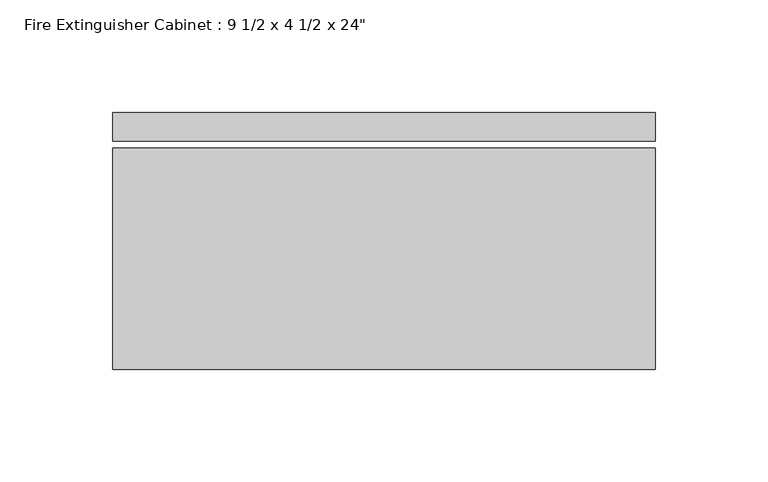
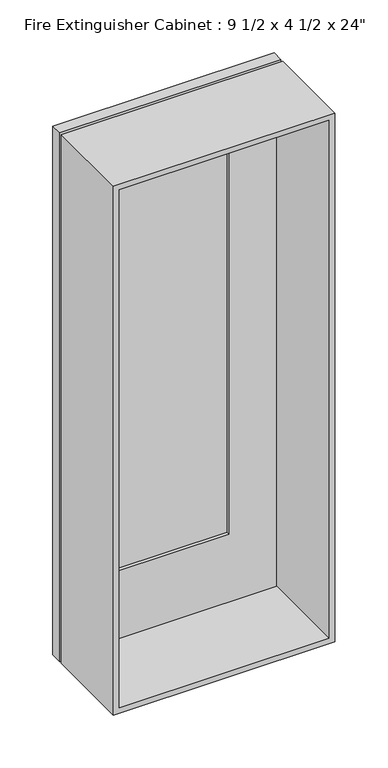
"""IFC4 building model written with IfcOpenShell, lengths in millimetres: proxy geometry."""

from ifc_helpers import new_model, si_unit, frame, origin, place, context, project, spatial, polyline, outline, extrude, source, transform, mapped, element, save


def proxy_8bb30bde(model_context):
    return source(origin(), model_context, "Body", "SweptSolid", [
        extrude(outline(polyline([(1524.0, -230.2984337), (914.4, -230.2984337), (914.4, 11.0015663), (1524.0, 11.0015663), (1524.0, -230.2984337)]), holes=[polyline([(1517.65, -223.9484337), (1517.65, 4.6515663), (920.75, 4.6515663), (920.75, -223.9484337), (1517.65, -223.9484337)])]), frame((0.0, 101.6, 0.0), z_axis=(0.0, 1.0, 0.0), x_axis=(0.0, 0.0, 1.0)), (0.0, 0.0, 1.0), 98.425),
        extrude(outline(polyline([(-173.1484337, 212.725), (-46.1484337, 212.725), (-46.1484337, 206.375), (-173.1484337, 206.375), (-173.1484337, 212.725)])), frame((0.0, 0.0, 996.95), z_axis=(0.0, 0.0, 1.0), x_axis=(1.0, 0.0, 0.0)), (0.0, 0.0, 1.0), 444.5),
        extrude(outline(polyline([(1524.0, -230.2984337), (914.4, -230.2984337), (914.4, 11.0015663), (1524.0, 11.0015663), (1524.0, -230.2984337)]), holes=[polyline([(1441.45, -173.1484337), (1441.45, -46.1484337), (996.95, -46.1484337), (996.95, -173.1484337), (1441.45, -173.1484337)])]), frame((0.0, 203.2, 0.0), z_axis=(0.0, 1.0, 0.0), x_axis=(0.0, 0.0, 1.0)), (0.0, 0.0, 1.0), 12.7),
    ])


if __name__ == "__main__":
    model = new_model("IFC4")
    model_context = context("Model", 3, world=origin())
    ifc_project = project(units=[si_unit("LENGTHUNIT", "METRE", prefix="MILLI")], contexts=[model_context])
    site = spatial("IfcSite", under=ifc_project)
    building = spatial("IfcBuilding", under=site)
    placement = place(None, origin())
    proxy_shape = proxy_8bb30bde(model_context)
    element("IfcBuildingElementProxy", 1, Name="Fire Extinguisher Cabinet : 9 1/2 x 4 1/2 x 24\"", ObjectType="Fire Extinguisher Cabinet : 9 1/2 x 4 1/2 x 24\"", at=placement, inside=building, context=model_context, shape_type="MappedRepresentation", body=[
        mapped(proxy_shape, transform((0.0, 0.0, 0.0), x_axis=(1.0, 0.0, 0.0), y_axis=(0.0, 1.0, 0.0), z_axis=(0.0, 0.0, 1.0))),
    ])
    save(model, "model.ifc")

# Revit data of these elements
# Type "Fire Extinguisher Cabinet : 9 1/2 x 4 1/2 x 24\""
#   Assembly Code = "D4030200"
#   Depth = 0' - 4 1/2"
#   Height = 2' - 0"
#   Mounting Height = 3' - 0"
#   Width = 0' - 9 1/2"
#   Cabinet Material = Metal - Paint Finish - Indian Red, Matte
#   Glass Pane Material = Glass
#   Default Elevation = 0
# Element 1 (IfcBuildingElementProxy, "Fire Extinguisher Cabinet : 9 1/2 x 4 1/2 x 24\"")
#   Materials on its faces: "Metal - Paint Finish - Indian Red, Matte", "Glass"
# Materials
#   "Metal - Paint Finish - Indian Red, Matte": class "Unassigned", colour RGB 114 47 47, transparency 0
#   "Glass": class "Unassigned", colour RGB 0 128 192, transparency 0.75, Description = "Glass"
